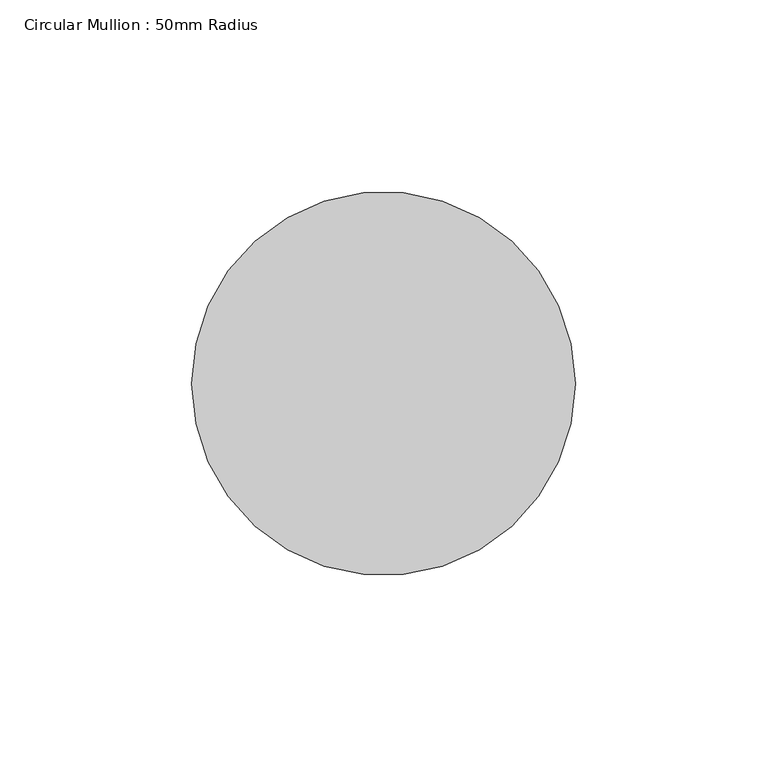
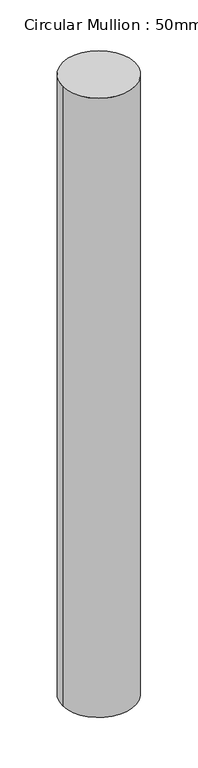
"""IFC4 building model written with IfcOpenShell, lengths in millimetres: member geometry, Circular Mullion : 50mm Radius."""

from ifc_helpers import new_model, si_unit, point, frame, origin, origin_2d, place, context, project, spatial, circle_curve, trimmed, segment, composite_curve, outline, extrude, source, transform, mapped, element, save


def circular_mullion_50mm_radius_c7faed01(model_context):
    return source(origin(), model_context, "Body", "SweptSolid", [
        extrude(outline(composite_curve([segment(trimmed(circle_curve(origin_2d(), 50.0), [point((50.0, 0.0))], [point((-50.0, 0.0))], False, "CARTESIAN"), True, "CONTINUOUS"), segment(trimmed(circle_curve(origin_2d(), 50.0), [point((-50.0, 0.0))], [point((50.0, 0.0))], False, "CARTESIAN"), True, "CONTINUOUS")], self_intersect=False)), frame((0.0, 0.0, -904.9398287), z_axis=(0.0, 0.0, 1.0), x_axis=(1.0, 0.0, 0.0)), (0.0, 0.0, 1.0), 904.9398287),
    ])


if __name__ == "__main__":
    model = new_model("IFC4")
    model_context = context("Model", 3, world=origin())
    ifc_project = project(units=[si_unit("LENGTHUNIT", "METRE", prefix="MILLI")], contexts=[model_context])
    site = spatial("IfcSite", under=ifc_project)
    building = spatial("IfcBuilding", under=site)
    placement = place(None, origin())
    circular_mullion_50mm_radius_shape = circular_mullion_50mm_radius_c7faed01(model_context)
    element("IfcMember", 1, ObjectType="Circular Mullion : 50mm Radius", at=placement, inside=building, context=model_context, shape_type="MappedRepresentation", body=[
        mapped(circular_mullion_50mm_radius_shape, transform((0.0, 0.0, 0.0), x_axis=(1.0, 0.0, 0.0), y_axis=(0.0, 1.0, 0.0), z_axis=(0.0, 0.0, 1.0))),
    ])
    save(model, "model.ifc")

# Revit data of these elements
# Type "Circular Mullion : 50mm Radius"
#   built-in parameter 1007350 = 0.164042 (stored number, unit not read)
# Element 1 (IfcMember, "Circular Mullion : 50mm Radius")
#   Materials on its faces: "Aluminium"
# Materials
#   "Aluminium": class "Metal", colour RGB 247 247 247, transparency 0, Description = "Aluminium 6061", Cost = 0
